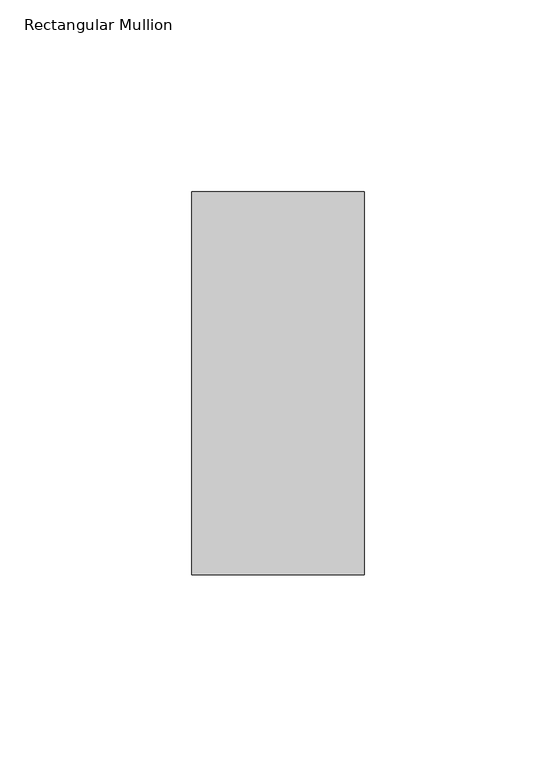
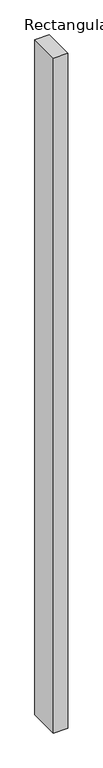
"""IFC4 building model written with IfcOpenShell, lengths in millimetres: member geometry, Rectangular Mullion : 알루미늄_Rectangular Cap_100 x 45."""

import ifcopenshell
import ifcopenshell.guid

model = None  # the IFC model being written
_history = None  # IfcOwnerHistory: only IFC2X3 demands one
_inside = {}  # id of a spatial element -> (the spatial element, [elements in it])
_under = {}  # id of a project, library or spatial element -> (it, [spatial elements below it])
_declared = {}  # id of a project -> (the project, [libraries it declares])
_typed = {}  # id of a type object -> (the type object, [elements of that type])
_made_of = {}  # id of a material, layer set ... -> (it, [elements and type objects made of it])


def new_model(schema):
    """Start an empty IFC model of exactly this schema.

    Asked for "IFC4X3", IfcOpenShell would pick the latest addendum, in which some entities
    have other attributes; the version numbers below select the first issue.
    IFC2X3 requires an IfcOwnerHistory on every rooted entity: one is made here for all.
    """
    global model, _history
    if schema == "IFC4X3":
        model = ifcopenshell.file(schema_version=(4, 3, 0, 0))
    else:
        model = ifcopenshell.file(schema=schema)
    _inside.clear()
    _under.clear()
    _declared.clear()
    _typed.clear()
    _made_of.clear()
    _history = None
    if model.schema == "IFC2X3":
        org = make("IfcOrganization", Name="unknown")
        user = make(
            "IfcPersonAndOrganization",
            ThePerson=make("IfcPerson", FamilyName="unknown"),
            TheOrganization=org,
        )
        app = make(
            "IfcApplication",
            ApplicationDeveloper=org,
            Version="unknown",
            ApplicationFullName="unknown",
            ApplicationIdentifier="unknown",
        )
        _history = make(
            "IfcOwnerHistory",
            OwningUser=user,
            OwningApplication=app,
            ChangeAction="ADDED",
            CreationDate=0,
        )
    return model


def make(cls, **values):
    """One entity of the class cls with the attributes given. An attribute that is None is left unset."""
    return model.create_entity(
        cls, **{name: value for name, value in values.items() if value is not None}
    )


def rooted(cls, **values):
    """An entity with a GlobalId (a new one), such as an element, a storey or a relation."""
    return make(cls, GlobalId=ifcopenshell.guid.new(), OwnerHistory=_history, **values)


def si_unit(unit_type, name, prefix=None):
    """IfcSIUnit, for example si_unit("LENGTHUNIT", "METRE", prefix="MILLI")."""
    return make("IfcSIUnit", UnitType=unit_type, Prefix=prefix, Name=name)


def assignment(units):
    """IfcUnitAssignment: the units of a project."""
    return None if units is None else make("IfcUnitAssignment", Units=units)


def point(xyz):
    """IfcCartesianPoint."""
    return None if xyz is None else make("IfcCartesianPoint", Coordinates=xyz)


def direction(xyz):
    """IfcDirection."""
    return None if xyz is None else make("IfcDirection", DirectionRatios=xyz)


def frame(location, z_axis=None, x_axis=None):
    """IfcAxis2Placement3D, a coordinate frame: its origin and axes. An axis left out is left unset."""
    return make(
        "IfcAxis2Placement3D",
        Location=point(location),
        Axis=direction(z_axis),
        RefDirection=direction(x_axis),
    )


def origin():
    """The frame at (0, 0, 0) with its axes left unset."""
    return frame((0.0, 0.0, 0.0))


def place(relative_to, where):
    """IfcLocalPlacement: puts the frame where relative to a parent placement (None: the world)."""
    return make(
        "IfcLocalPlacement", PlacementRelTo=relative_to, RelativePlacement=where
    )


def context(
    kind, dimensions, precision=None, world=None, true_north=None, identifier=None
):
    """IfcGeometricRepresentationContext, for example the 3D "Model" context."""
    return make(
        "IfcGeometricRepresentationContext",
        ContextIdentifier=identifier,
        ContextType=kind,
        CoordinateSpaceDimension=dimensions,
        Precision=precision,
        WorldCoordinateSystem=world,
        TrueNorth=true_north,
    )


def project(units=None, contexts=None):
    """IfcProject with its units and contexts."""
    return rooted(
        "IfcProject",
        Name="project",
        RepresentationContexts=contexts,
        UnitsInContext=assignment(units),
    )


def spatial(cls, under=None, at=None, **own):
    """A site, building, storey or space (cls), placed at a placement, below another one or the project."""
    s = rooted(cls, ObjectPlacement=at, **own)
    if under is not None:
        _under.setdefault(under.id(), (under, []))[1].append(s)
    return s


def polyline(points):
    """IfcPolyline through the points."""
    return make("IfcPolyline", Points=[point(p) for p in points])


def outline(outer, holes=None, kind="AREA"):
    """IfcArbitraryClosedProfileDef: a profile drawn as a closed curve; with holes, ...WithVoids."""
    if holes is None:
        return make("IfcArbitraryClosedProfileDef", ProfileType=kind, OuterCurve=outer)
    return make(
        "IfcArbitraryProfileDefWithVoids",
        ProfileType=kind,
        OuterCurve=outer,
        InnerCurves=holes,
    )


def extrude(swept, where, along, depth):
    """IfcExtrudedAreaSolid: the profile swept, set in the frame where, extruded along a direction by depth."""
    return make(
        "IfcExtrudedAreaSolid",
        SweptArea=swept,
        Position=where,
        ExtrudedDirection=direction(along),
        Depth=depth,
    )


def shape(context_of_items, identifier, shape_type, items):
    """IfcShapeRepresentation: the items that make up one representation, for example the "Body"."""
    return make(
        "IfcShapeRepresentation",
        ContextOfItems=context_of_items,
        RepresentationIdentifier=identifier,
        RepresentationType=shape_type,
        Items=items,
    )


def source(mapping_origin, context_of_items, identifier, shape_type, items):
    """IfcRepresentationMap: a shape defined once, which mapped items show again and again."""
    return make(
        "IfcRepresentationMap",
        MappingOrigin=mapping_origin,
        MappedRepresentation=shape(context_of_items, identifier, shape_type, items),
    )


def transform(
    local_origin,
    x_axis=None,
    y_axis=None,
    z_axis=None,
    scale=None,
    scale2=None,
    scale3=None,
    uniform=True,
):
    """IfcCartesianTransformationOperator3D, or its non-uniform kind. x_axis, y_axis, z_axis: its Axis1, 2, 3."""
    if uniform:
        return make(
            "IfcCartesianTransformationOperator3D",
            Axis1=direction(x_axis),
            Axis2=direction(y_axis),
            LocalOrigin=point(local_origin),
            Scale=scale,
            Axis3=direction(z_axis),
        )
    return make(
        "IfcCartesianTransformationOperator3DnonUniform",
        Axis1=direction(x_axis),
        Axis2=direction(y_axis),
        LocalOrigin=point(local_origin),
        Scale=scale,
        Axis3=direction(z_axis),
        Scale2=scale2,
        Scale3=scale3,
    )


def mapped(mapping_source, mapping_target):
    """IfcMappedItem: shows the shape of a source again, moved by a transform."""
    return make(
        "IfcMappedItem", MappingSource=mapping_source, MappingTarget=mapping_target
    )


def made_of(thing, what):
    """Note that an element or type object is made of a material, layer set ...; save() writes the relation."""
    if what is not None:
        _made_of.setdefault(what.id(), (what, []))[1].append(thing)
    return thing


def element(
    cls,
    number,
    at=None,
    inside=None,
    cuts=None,
    type_object=None,
    material=None,
    context=None,
    identifier="Body",
    shape_type=None,
    held_by="IfcProductDefinitionShape",
    body=None,
    shapes=None,
    **own,
):
    """One element of the class cls, such as IfcWall. Its Tag is "e" and its number.

    at: its placement. inside: the storey or other place that contains it. cuts: it is an
    opening in that element (IfcRelVoidsElement). A single representation is given by context,
    identifier, shape_type and body (its items); several are given by shapes. held_by: the class
    of the entity that holds the representations. save() writes the other relations.
    """
    e = rooted(cls, Tag="e%d" % number, ObjectPlacement=at, **own)
    if body is not None:
        shapes = [shape(context, identifier, shape_type, body)]
    if shapes is not None:
        e.Representation = make(held_by, Representations=shapes)
    if inside is not None:
        _inside.setdefault(inside.id(), (inside, []))[1].append(e)
    if cuts is not None:
        rooted(
            "IfcRelVoidsElement", RelatingBuildingElement=cuts, RelatedOpeningElement=e
        )
    if type_object is not None:
        _typed.setdefault(type_object.id(), (type_object, []))[1].append(e)
    return made_of(e, material)


def aggregate(whole, parts):
    """IfcRelAggregates: a whole, such as a stair, and the parts it consists of."""
    return rooted("IfcRelAggregates", RelatingObject=whole, RelatedObjects=parts)


def save(model, path):
    """Write the relations noted so far, then the file.

    IfcRelAggregates (storeys below a building ...), IfcRelContainedInSpatialStructure (elements
    in a storey), IfcRelDefinesByType, IfcRelAssociatesMaterial and IfcRelDeclares: one each for
    every whole, place, type object, material and project.
    """
    for whole, parts in _under.values():
        aggregate(whole, parts)
    for where, things in _inside.values():
        rooted(
            "IfcRelContainedInSpatialStructure",
            RelatedElements=things,
            RelatingStructure=where,
        )
    for kind, things in _typed.values():
        rooted("IfcRelDefinesByType", RelatedObjects=things, RelatingType=kind)
    for what, things in _made_of.values():
        rooted("IfcRelAssociatesMaterial", RelatedObjects=things, RelatingMaterial=what)
    for by, libraries in _declared.values():
        rooted("IfcRelDeclares", RelatingContext=by, RelatedDefinitions=libraries)
    model.write(path)


def rectangular_mullion_3ef7a803(model_context):
    return source(origin(), model_context, "Body", "SweptSolid", [
        extrude(outline(polyline([(22.5, 50.0), (22.5, -50.0), (-22.5, -50.0), (-22.5, 50.0), (22.5, 50.0)])), frame((0.0, 0.0, -2222.5), z_axis=(0.0, 0.0, 1.0), x_axis=(1.0, 0.0, 0.0)), (0.0, 0.0, 1.0), 2222.5),
    ])


if __name__ == "__main__":
    model = new_model("IFC4")
    model_context = context("Model", 3, world=origin())
    ifc_project = project(units=[si_unit("LENGTHUNIT", "METRE", prefix="MILLI")], contexts=[model_context])
    site = spatial("IfcSite", under=ifc_project)
    building = spatial("IfcBuilding", under=site)
    placement = place(None, origin())
    rectangular_mullion_shape = rectangular_mullion_3ef7a803(model_context)
    element("IfcMember", 1, ObjectType="Rectangular Mullion : 알루미늄_Rectangular Cap_100 x 45", at=placement, inside=building, context=model_context, shape_type="MappedRepresentation", body=[
        mapped(rectangular_mullion_shape, transform((0.0, 0.0, 0.0), x_axis=(1.0, 0.0, 0.0), y_axis=(0.0, 1.0, 0.0), z_axis=(0.0, 0.0, 1.0))),
    ])
    save(model, "model.ifc")

# Revit data of these elements
# Type "Rectangular Mullion : 알루미늄_Rectangular Cap_100 x 45"
#   built-in parameter 1007304 = 0.328084 (stored number, unit not read)
#   built-in parameter 1007301 = 0.0738189 (stored number, unit not read)
#   built-in parameter 1007300 = 0.0738189 (stored number, unit not read)
# Element 1 (IfcMember, "Rectangular Mullion : 알루미늄_Rectangular Cap_100 x 45")
#   Materials on its faces: "00_Metal_Stainless Steel"
# Materials
#   "00_Metal_Stainless Steel": class "Metal", colour RGB 148 148 148, transparency 0, Description = "Steel", Cost = 0
